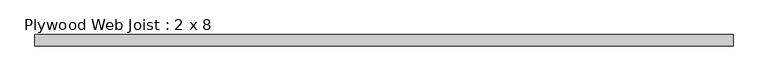
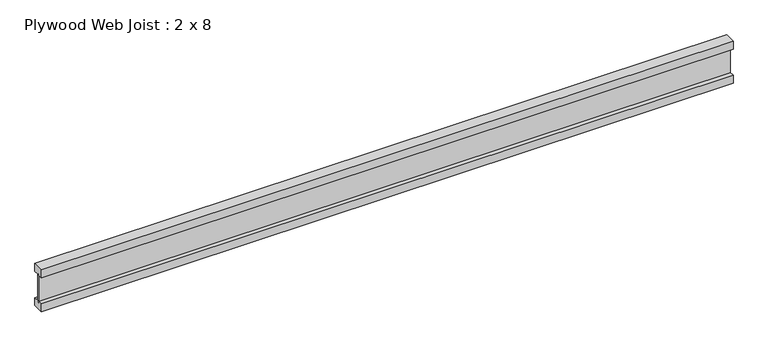
"""IFC4 building model written with IfcOpenShell, lengths in millimetres: beam geometry, Plywood Web Joist : 2 x 8."""

import ifcopenshell
import ifcopenshell.guid

model = None  # the IFC model being written
_history = None  # IfcOwnerHistory: only IFC2X3 demands one
_inside = {}  # id of a spatial element -> (the spatial element, [elements in it])
_under = {}  # id of a project, library or spatial element -> (it, [spatial elements below it])
_declared = {}  # id of a project -> (the project, [libraries it declares])
_typed = {}  # id of a type object -> (the type object, [elements of that type])
_made_of = {}  # id of a material, layer set ... -> (it, [elements and type objects made of it])


def new_model(schema):
    """Start an empty IFC model of exactly this schema.

    Asked for "IFC4X3", IfcOpenShell would pick the latest addendum, in which some entities
    have other attributes; the version numbers below select the first issue.
    IFC2X3 requires an IfcOwnerHistory on every rooted entity: one is made here for all.
    """
    global model, _history
    if schema == "IFC4X3":
        model = ifcopenshell.file(schema_version=(4, 3, 0, 0))
    else:
        model = ifcopenshell.file(schema=schema)
    _inside.clear()
    _under.clear()
    _declared.clear()
    _typed.clear()
    _made_of.clear()
    _history = None
    if model.schema == "IFC2X3":
        org = make("IfcOrganization", Name="unknown")
        user = make(
            "IfcPersonAndOrganization",
            ThePerson=make("IfcPerson", FamilyName="unknown"),
            TheOrganization=org,
        )
        app = make(
            "IfcApplication",
            ApplicationDeveloper=org,
            Version="unknown",
            ApplicationFullName="unknown",
            ApplicationIdentifier="unknown",
        )
        _history = make(
            "IfcOwnerHistory",
            OwningUser=user,
            OwningApplication=app,
            ChangeAction="ADDED",
            CreationDate=0,
        )
    return model


def make(cls, **values):
    """One entity of the class cls with the attributes given. An attribute that is None is left unset."""
    return model.create_entity(
        cls, **{name: value for name, value in values.items() if value is not None}
    )


def rooted(cls, **values):
    """An entity with a GlobalId (a new one), such as an element, a storey or a relation."""
    return make(cls, GlobalId=ifcopenshell.guid.new(), OwnerHistory=_history, **values)


def si_unit(unit_type, name, prefix=None):
    """IfcSIUnit, for example si_unit("LENGTHUNIT", "METRE", prefix="MILLI")."""
    return make("IfcSIUnit", UnitType=unit_type, Prefix=prefix, Name=name)


def assignment(units):
    """IfcUnitAssignment: the units of a project."""
    return None if units is None else make("IfcUnitAssignment", Units=units)


def point(xyz):
    """IfcCartesianPoint."""
    return None if xyz is None else make("IfcCartesianPoint", Coordinates=xyz)


def direction(xyz):
    """IfcDirection."""
    return None if xyz is None else make("IfcDirection", DirectionRatios=xyz)


def frame(location, z_axis=None, x_axis=None):
    """IfcAxis2Placement3D, a coordinate frame: its origin and axes. An axis left out is left unset."""
    return make(
        "IfcAxis2Placement3D",
        Location=point(location),
        Axis=direction(z_axis),
        RefDirection=direction(x_axis),
    )


def origin():
    """The frame at (0, 0, 0) with its axes left unset."""
    return frame((0.0, 0.0, 0.0))


def place(relative_to, where):
    """IfcLocalPlacement: puts the frame where relative to a parent placement (None: the world)."""
    return make(
        "IfcLocalPlacement", PlacementRelTo=relative_to, RelativePlacement=where
    )


def context(
    kind, dimensions, precision=None, world=None, true_north=None, identifier=None
):
    """IfcGeometricRepresentationContext, for example the 3D "Model" context."""
    return make(
        "IfcGeometricRepresentationContext",
        ContextIdentifier=identifier,
        ContextType=kind,
        CoordinateSpaceDimension=dimensions,
        Precision=precision,
        WorldCoordinateSystem=world,
        TrueNorth=true_north,
    )


def project(units=None, contexts=None):
    """IfcProject with its units and contexts."""
    return rooted(
        "IfcProject",
        Name="project",
        RepresentationContexts=contexts,
        UnitsInContext=assignment(units),
    )


def spatial(cls, under=None, at=None, **own):
    """A site, building, storey or space (cls), placed at a placement, below another one or the project."""
    s = rooted(cls, ObjectPlacement=at, **own)
    if under is not None:
        _under.setdefault(under.id(), (under, []))[1].append(s)
    return s


def polyline(points):
    """IfcPolyline through the points."""
    return make("IfcPolyline", Points=[point(p) for p in points])


def outline(outer, holes=None, kind="AREA"):
    """IfcArbitraryClosedProfileDef: a profile drawn as a closed curve; with holes, ...WithVoids."""
    if holes is None:
        return make("IfcArbitraryClosedProfileDef", ProfileType=kind, OuterCurve=outer)
    return make(
        "IfcArbitraryProfileDefWithVoids",
        ProfileType=kind,
        OuterCurve=outer,
        InnerCurves=holes,
    )


def extrude(swept, where, along, depth):
    """IfcExtrudedAreaSolid: the profile swept, set in the frame where, extruded along a direction by depth."""
    return make(
        "IfcExtrudedAreaSolid",
        SweptArea=swept,
        Position=where,
        ExtrudedDirection=direction(along),
        Depth=depth,
    )


def shape(context_of_items, identifier, shape_type, items):
    """IfcShapeRepresentation: the items that make up one representation, for example the "Body"."""
    return make(
        "IfcShapeRepresentation",
        ContextOfItems=context_of_items,
        RepresentationIdentifier=identifier,
        RepresentationType=shape_type,
        Items=items,
    )


def source(mapping_origin, context_of_items, identifier, shape_type, items):
    """IfcRepresentationMap: a shape defined once, which mapped items show again and again."""
    return make(
        "IfcRepresentationMap",
        MappingOrigin=mapping_origin,
        MappedRepresentation=shape(context_of_items, identifier, shape_type, items),
    )


def transform(
    local_origin,
    x_axis=None,
    y_axis=None,
    z_axis=None,
    scale=None,
    scale2=None,
    scale3=None,
    uniform=True,
):
    """IfcCartesianTransformationOperator3D, or its non-uniform kind. x_axis, y_axis, z_axis: its Axis1, 2, 3."""
    if uniform:
        return make(
            "IfcCartesianTransformationOperator3D",
            Axis1=direction(x_axis),
            Axis2=direction(y_axis),
            LocalOrigin=point(local_origin),
            Scale=scale,
            Axis3=direction(z_axis),
        )
    return make(
        "IfcCartesianTransformationOperator3DnonUniform",
        Axis1=direction(x_axis),
        Axis2=direction(y_axis),
        LocalOrigin=point(local_origin),
        Scale=scale,
        Axis3=direction(z_axis),
        Scale2=scale2,
        Scale3=scale3,
    )


def mapped(mapping_source, mapping_target):
    """IfcMappedItem: shows the shape of a source again, moved by a transform."""
    return make(
        "IfcMappedItem", MappingSource=mapping_source, MappingTarget=mapping_target
    )


def made_of(thing, what):
    """Note that an element or type object is made of a material, layer set ...; save() writes the relation."""
    if what is not None:
        _made_of.setdefault(what.id(), (what, []))[1].append(thing)
    return thing


def element(
    cls,
    number,
    at=None,
    inside=None,
    cuts=None,
    type_object=None,
    material=None,
    context=None,
    identifier="Body",
    shape_type=None,
    held_by="IfcProductDefinitionShape",
    body=None,
    shapes=None,
    **own,
):
    """One element of the class cls, such as IfcWall. Its Tag is "e" and its number.

    at: its placement. inside: the storey or other place that contains it. cuts: it is an
    opening in that element (IfcRelVoidsElement). A single representation is given by context,
    identifier, shape_type and body (its items); several are given by shapes. held_by: the class
    of the entity that holds the representations. save() writes the other relations.
    """
    e = rooted(cls, Tag="e%d" % number, ObjectPlacement=at, **own)
    if body is not None:
        shapes = [shape(context, identifier, shape_type, body)]
    if shapes is not None:
        e.Representation = make(held_by, Representations=shapes)
    if inside is not None:
        _inside.setdefault(inside.id(), (inside, []))[1].append(e)
    if cuts is not None:
        rooted(
            "IfcRelVoidsElement", RelatingBuildingElement=cuts, RelatedOpeningElement=e
        )
    if type_object is not None:
        _typed.setdefault(type_object.id(), (type_object, []))[1].append(e)
    return made_of(e, material)


def aggregate(whole, parts):
    """IfcRelAggregates: a whole, such as a stair, and the parts it consists of."""
    return rooted("IfcRelAggregates", RelatingObject=whole, RelatedObjects=parts)


def save(model, path):
    """Write the relations noted so far, then the file.

    IfcRelAggregates (storeys below a building ...), IfcRelContainedInSpatialStructure (elements
    in a storey), IfcRelDefinesByType, IfcRelAssociatesMaterial and IfcRelDeclares: one each for
    every whole, place, type object, material and project.
    """
    for whole, parts in _under.values():
        aggregate(whole, parts)
    for where, things in _inside.values():
        rooted(
            "IfcRelContainedInSpatialStructure",
            RelatedElements=things,
            RelatingStructure=where,
        )
    for kind, things in _typed.values():
        rooted("IfcRelDefinesByType", RelatedObjects=things, RelatingType=kind)
    for what, things in _made_of.values():
        rooted("IfcRelAssociatesMaterial", RelatedObjects=things, RelatingMaterial=what)
    for by, libraries in _declared.values():
        rooted("IfcRelDeclares", RelatingContext=by, RelatedDefinitions=libraries)
    model.write(path)


def plywood_web_joist_2_x_8_5f52603e(model_context):
    return source(origin(), model_context, "Body", "SweptSolid", [
        extrude(outline(polyline([(-25.4, 101.6), (25.4, 101.6), (25.4, 63.5), (4.7625, 63.5), (4.7625, 69.85), (-4.7625, 69.85), (-4.7625, 63.5), (-25.4, 63.5), (-25.4, 101.6)])), frame((-1584.325, 0.0, 0.0), z_axis=(1.0, 0.0, 0.0), x_axis=(0.0, 1.0, 0.0)), (0.0, 0.0, 1.0), 3168.65),
        extrude(outline(polyline([(25.4, -63.5), (25.4, -101.6), (-25.4, -101.6), (-25.4, -63.5), (-4.7625, -63.5), (-4.7625, -69.1160374), (4.7625, -69.1160374), (4.7625, -63.5), (25.4, -63.5)])), frame((-1584.325, 0.0, 0.0), z_axis=(1.0, 0.0, 0.0), x_axis=(0.0, 1.0, 0.0)), (0.0, 0.0, 1.0), 3168.65),
        extrude(outline(polyline([(1584.325, 4.7625), (1584.325, -4.7625), (-1584.325, -4.7625), (-1584.325, 4.7625), (1584.325, 4.7625)])), frame((0.0, 0.0, -69.1160374), z_axis=(0.0, 0.0, 1.0), x_axis=(1.0, 0.0, 0.0)), (0.0, 0.0, 1.0), 138.9660374),
    ])


if __name__ == "__main__":
    model = new_model("IFC4")
    model_context = context("Model", 3, world=origin())
    ifc_project = project(units=[si_unit("LENGTHUNIT", "METRE", prefix="MILLI")], contexts=[model_context])
    site = spatial("IfcSite", under=ifc_project)
    building = spatial("IfcBuilding", under=site)
    placement = place(None, origin())
    plywood_web_joist_2_x_8_shape = plywood_web_joist_2_x_8_5f52603e(model_context)
    element("IfcBeam", 1, ObjectType="Plywood Web Joist : 2 x 8", at=placement, inside=building, context=model_context, shape_type="MappedRepresentation", body=[
        mapped(plywood_web_joist_2_x_8_shape, transform((0.0, 0.0, 0.0), x_axis=(1.0, 0.0, 0.0), y_axis=(0.0, 1.0, 0.0), z_axis=(0.0, 0.0, 1.0))),
    ])
    save(model, "model.ifc")

# Revit data of these elements
# Type "Plywood Web Joist : 2 x 8"
#   Assembly Code = "B10"
#   Length [instance default] = 5' - 0"
#   b = 0' - 2"
#   d = 0' - 8"
#   Structural Material [instance default] = Softwood, Lumber
# Element 1 (IfcBeam, "Plywood Web Joist : 2 x 8")
#   Materials on its faces: "Softwood, Lumber"
# Materials
#   "Softwood, Lumber": class "Wood", colour RGB 144 113 62, transparency 0, Description = "Pinus Echinata", Cost = 0
